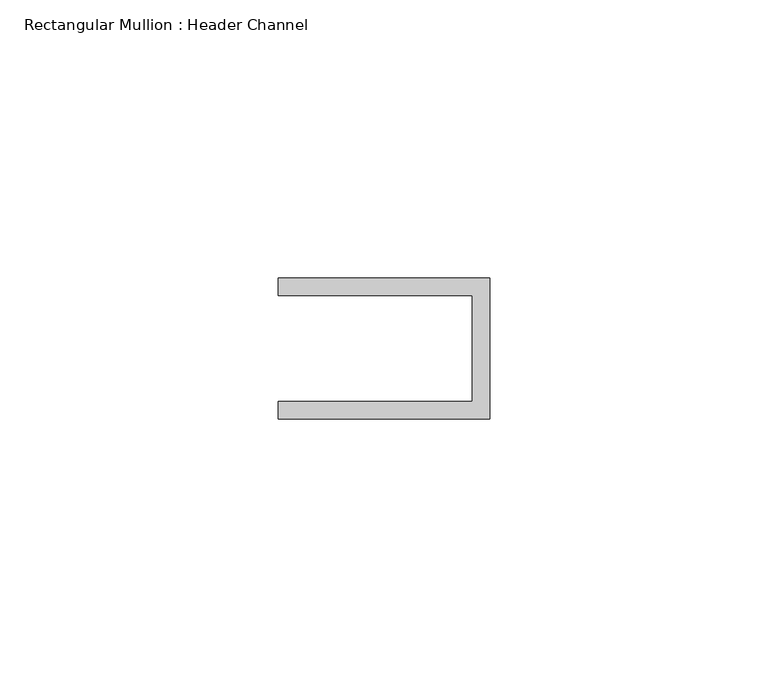
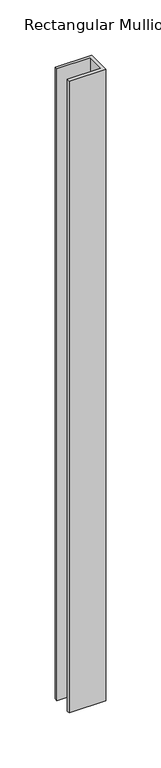
"""IFC4 building model written with IfcOpenShell, lengths in millimetres: member geometry, Rectangular Mullion : Header Channel."""

from ifc_helpers import new_model, si_unit, frame, origin, place, context, project, spatial, polyline, outline, extrude, source, transform, mapped, element, save


def rectangular_mullion_header_channel_6ccc843e(model_context):
    return source(origin(), model_context, "Body", "SweptSolid", [
        extrude(outline(polyline([(0.0, -12.7), (-38.1, -12.7), (-38.1, -9.525), (-3.175, -9.525), (-3.175, 9.525), (-38.1, 9.525), (-38.1, 12.7), (0.0, 12.7), (0.0, -12.7)])), frame((0.0, 0.0, -698.5), z_axis=(0.0, 0.0, 1.0), x_axis=(1.0, 0.0, 0.0)), (0.0, 0.0, 1.0), 698.5),
    ])


if __name__ == "__main__":
    model = new_model("IFC4")
    model_context = context("Model", 3, world=origin())
    ifc_project = project(units=[si_unit("LENGTHUNIT", "METRE", prefix="MILLI")], contexts=[model_context])
    site = spatial("IfcSite", under=ifc_project)
    building = spatial("IfcBuilding", under=site)
    placement = place(None, origin())
    rectangular_mullion_header_channel_shape = rectangular_mullion_header_channel_6ccc843e(model_context)
    element("IfcMember", 1, ObjectType="Rectangular Mullion : Header Channel", at=placement, inside=building, context=model_context, shape_type="MappedRepresentation", body=[
        mapped(rectangular_mullion_header_channel_shape, transform((0.0, 0.0, 0.0), x_axis=(1.0, 0.0, 0.0), y_axis=(0.0, 1.0, 0.0), z_axis=(0.0, 0.0, 1.0))),
    ])
    save(model, "model.ifc")

# Revit data of these elements
# Type "Rectangular Mullion : Header Channel"
#   built-in parameter 1007322 = 0.0833333 (stored number, unit not read)
#   built-in parameter 1007321 = -0.03125 (stored number, unit not read)
#   built-in parameter 1007320 = 0.0416667 (stored number, unit not read)
# Element 1 (IfcMember, "Rectangular Mullion : Header Channel")
#   Materials on its faces: "ALUM"
# Materials
#   "ALUM": class "Generic", colour RGB 157 157 157, transparency 0, Cost = 0
